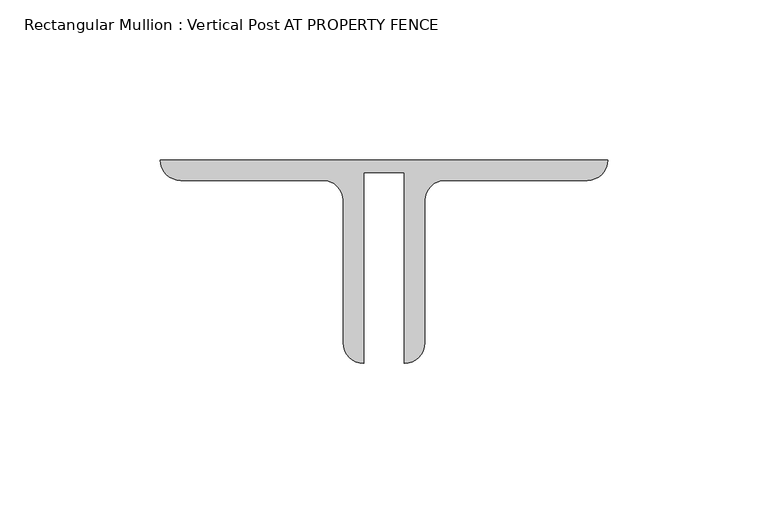
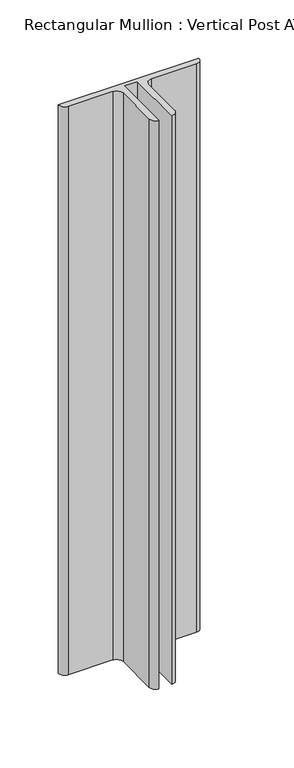
"""IFC4 building model written with IfcOpenShell, lengths in millimetres: member geometry, Rectangular Mullion : Vertical Post AT PROPERTY FENCE."""

from ifc_helpers import new_model, si_unit, point, frame, frame_2d, origin, place, context, project, spatial, polyline, circle_curve, trimmed, segment, composite_curve, outline, extrude, source, transform, mapped, element, save


def rectangular_mullion_vertical_post_at_property_fence_4eff7762(model_context):
    return source(origin(), model_context, "Body", "SweptSolid", [
        extrude(outline(composite_curve([segment(polyline([(-76.2, -22.9145205), (-76.2, -82.55)]), True, "CONTINUOUS"), segment(trimmed(circle_curve(frame_2d((-76.2, -76.2)), 6.35), [point((-76.2, -82.55))], [point((-82.55, -76.2))], False, "CARTESIAN"), True, "CONTINUOUS"), segment(polyline([(-82.55, -76.2), (-82.55, -31.75)]), True, "CONTINUOUS"), segment(trimmed(circle_curve(frame_2d((-88.9, -31.75)), 6.35), [point((-82.55, -31.75))], [point((-88.9, -25.4))], True, "CARTESIAN"), True, "CONTINUOUS"), segment(polyline([(-88.9, -25.4), (-133.35, -25.4)]), True, "CONTINUOUS"), segment(trimmed(circle_curve(frame_2d((-133.35, -19.05)), 6.35), [point((-133.35, -25.4))], [point((-139.7, -19.05))], False, "CARTESIAN"), True, "CONTINUOUS"), segment(polyline([(-139.7, -19.05), (0.0, -19.05)]), True, "CONTINUOUS"), segment(trimmed(circle_curve(frame_2d((-6.35, -19.05)), 6.35), [point((0.0, -19.05))], [point((-6.35, -25.4))], False, "CARTESIAN"), True, "CONTINUOUS"), segment(polyline([(-6.35, -25.4), (-50.8, -25.4)]), True, "CONTINUOUS"), segment(trimmed(circle_curve(frame_2d((-50.8, -31.75)), 6.35), [point((-50.8, -25.4))], [point((-57.15, -31.75))], True, "CARTESIAN"), True, "CONTINUOUS"), segment(polyline([(-57.15, -31.75), (-57.15, -76.2)]), True, "CONTINUOUS"), segment(trimmed(circle_curve(frame_2d((-63.5, -76.2)), 6.35), [point((-57.15, -76.2))], [point((-63.5, -82.55))], False, "CARTESIAN"), True, "CONTINUOUS"), segment(polyline([(-63.5, -82.55), (-63.5, -22.9145205), (-76.2, -22.9145205)]), True, "CONTINUOUS")], self_intersect=False)), frame((0.0, 0.0, -596.9), z_axis=(0.0, 0.0, 1.0), x_axis=(1.0, 0.0, 0.0)), (0.0, 0.0, 1.0), 596.9),
    ])


if __name__ == "__main__":
    model = new_model("IFC4")
    model_context = context("Model", 3, world=origin())
    ifc_project = project(units=[si_unit("LENGTHUNIT", "METRE", prefix="MILLI")], contexts=[model_context])
    site = spatial("IfcSite", under=ifc_project)
    building = spatial("IfcBuilding", under=site)
    placement = place(None, origin())
    rectangular_mullion_vertical_post_at_property_fence_shape = rectangular_mullion_vertical_post_at_property_fence_4eff7762(model_context)
    element("IfcMember", 1, ObjectType="Rectangular Mullion : Vertical Post AT PROPERTY FENCE", at=placement, inside=building, context=model_context, shape_type="MappedRepresentation", body=[
        mapped(rectangular_mullion_vertical_post_at_property_fence_shape, transform((0.0, 0.0, 0.0), x_axis=(1.0, 0.0, 0.0), y_axis=(0.0, 1.0, 0.0), z_axis=(0.0, 0.0, 1.0))),
    ])
    save(model, "model.ifc")

# Revit data of these elements
# Type "Rectangular Mullion : Vertical Post AT PROPERTY FENCE"
#   built-in parameter 1007351 = -0.0625 (stored number, unit not read)
#   built-in parameter 1007322 = 0.0126789 (stored number, unit not read)
#   built-in parameter 1007321 = 0.229167 (stored number, unit not read)
#   built-in parameter 1007320 = 0.229167 (stored number, unit not read)
# Element 1 (IfcMember, "Rectangular Mullion : Vertical Post AT PROPERTY FENCE")
#   Materials on its faces: "MAIN FENCE POST: (2) BACK/BACK GALVANIZED ANGLES (2) L2 1/2 X 2 1/2 X 1/4\") ANCHORED TO 8\"W X 42\" DEEP CONCRETE FOOTING(1)"
# Materials
#   "MAIN FENCE POST: (2) BACK/BACK GALVANIZED ANGLES (2) L2 1/2 X 2 1/2 X 1/4\") ANCHORED TO 8\"W X 42\" DEEP CONCRETE FOOTING(1)": class "Unassigned", colour RGB 211 211 211, transparency 0, Cost = 0
